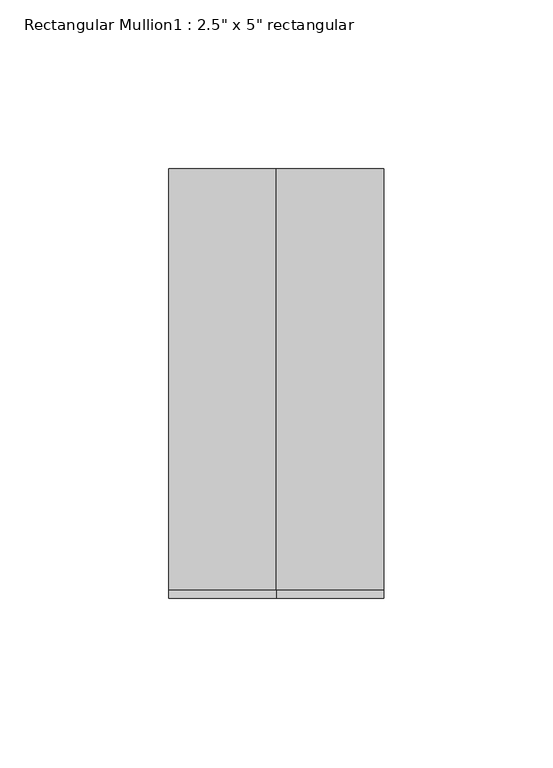
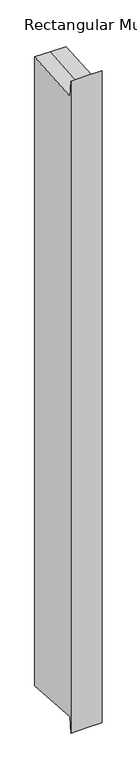
"""IFC4 building model written with IfcOpenShell, lengths in millimetres: member geometry."""

from ifc_helpers import new_model, si_unit, origin, place, context, project, spatial, faceted_brep, source, transform, mapped, element, save


def member_995572cb(model_context):
    return source(origin(), model_context, "Body", "Brep", [
        faceted_brep([(-31.75, 63.5, 4.5282284), (0.0, 63.5, 4.5282284), (31.75, 63.5, 4.5282284), (31.75, 63.5, -1343.9489353), (0.0, 63.5, -1343.9489353), (-31.75, 63.5, -1343.9489353), (-31.75, -63.5, 29.4471051), (-31.75, -61.0333155, -4.5163328), (-31.75, -61.0333155, -1334.904374), (-31.75, -63.5, -1368.8678119), (31.75, -63.5, 29.4471051), (0.0, -63.5, 29.4471051), (0.0, -63.5, -1368.8678119), (31.75, -63.5, -1368.8678119), (31.75, -61.0333155, -4.5163328), (31.75, -61.0333155, -1334.904374), (0.0, -61.0333155, -4.5163328), (0.0, -61.0333155, -1334.904374)], [[[0, 1, 2, 3, 4, 5]], [[6, 7, 0, 5, 8, 9]], [[10, 11, 6, 9, 12, 13]], [[2, 14, 10, 13, 15, 3]], [[2, 1, 16, 14]], [[1, 0, 7, 16]], [[7, 6, 11, 16]], [[11, 10, 14, 16]], [[3, 15, 17, 4]], [[15, 13, 12, 17]], [[12, 9, 8, 17]], [[8, 5, 4, 17]]]),
    ])


if __name__ == "__main__":
    model = new_model("IFC4")
    model_context = context("Model", 3, world=origin())
    ifc_project = project(units=[si_unit("LENGTHUNIT", "METRE", prefix="MILLI")], contexts=[model_context])
    site = spatial("IfcSite", under=ifc_project)
    building = spatial("IfcBuilding", under=site)
    placement = place(None, origin())
    member_shape = member_995572cb(model_context)
    element("IfcMember", 1, ObjectType="Rectangular Mullion1 : 2.5\" x 5\" rectangular", at=placement, inside=building, context=model_context, shape_type="MappedRepresentation", body=[
        mapped(member_shape, transform((0.0, 0.0, 0.0), x_axis=(1.0, 0.0, 0.0), y_axis=(0.0, 1.0, 0.0), z_axis=(0.0, 0.0, 1.0))),
    ])
    save(model, "model.ifc")

# Revit data of these elements
# Type "Rectangular Mullion1 : 2.5\" x 5\" rectangular"
#   built-in parameter 1007304 = 0.416667 (stored number, unit not read)
#   built-in parameter 1007301 = 0.104167 (stored number, unit not read)
#   built-in parameter 1007300 = 0.104167 (stored number, unit not read)
# Element 1 (IfcMember, "Rectangular Mullion1 : 2.5\" x 5\" rectangular")
#   Materials on its faces: "support-frame"
# Materials
#   "support-frame": class "Unassigned", colour RGB 233 233 233, transparency 0, Cost = 0
